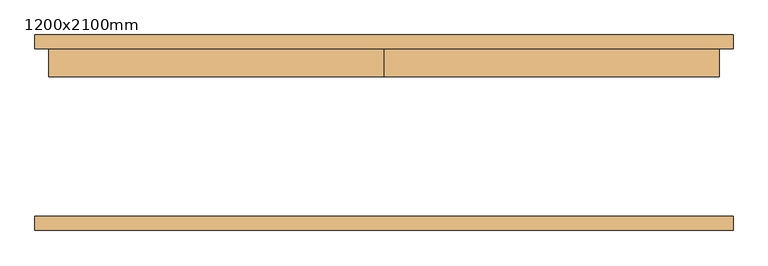
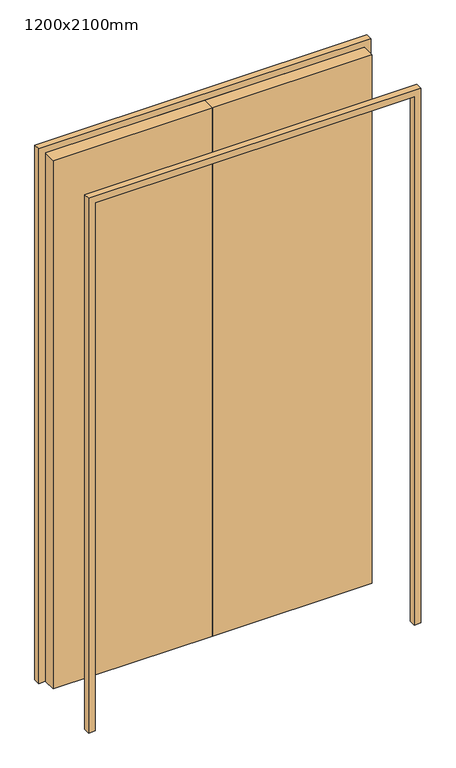
"""IFC4 building model written with IfcOpenShell, lengths in millimetres: door geometry, WWm-DoubleSolid-Flush : 1200x2100mm."""

from ifc_helpers import new_model, si_unit, frame, origin, origin_with_axes, place, context, project, spatial, polyline, outline, extrude, source, transform, mapped, element, save


def door_1200x2100mm_805ceeaa(model_context):
    return source(origin(), model_context, "Body", "SweptSolid", [
        extrude(outline(polyline([(0.0, 150.0), (600.0, 150.0), (600.0, 100.0), (0.0, 100.0), (0.0, 150.0)])), origin_with_axes(), (0.0, 0.0, 1.0), 2100.0),
        extrude(outline(polyline([(-600.0, 150.0), (0.0, 150.0), (0.0, 100.0), (-600.0, 100.0), (-600.0, 150.0)])), origin_with_axes(), (0.0, 0.0, 1.0), 2100.0),
        extrude(outline(polyline([(2100.0, -600.0), (2100.0, 600.0), (0.0, 600.0), (0.0, 625.0), (2125.0, 625.0), (2125.0, -625.0), (0.0, -625.0), (0.0, -600.0), (2100.0, -600.0)])), frame((0.0, -175.0, 0.0), z_axis=(0.0, 1.0, 0.0), x_axis=(0.0, 0.0, 1.0)), (0.0, 0.0, 1.0), 25.0),
        extrude(outline(polyline([(2100.0, -600.0), (2100.0, 600.0), (0.0, 600.0), (0.0, 625.0), (2125.0, 625.0), (2125.0, -625.0), (0.0, -625.0), (0.0, -600.0), (2100.0, -600.0)])), frame((0.0, 150.0, 0.0), z_axis=(0.0, 1.0, 0.0), x_axis=(0.0, 0.0, 1.0)), (0.0, 0.0, 1.0), 25.0),
    ])


if __name__ == "__main__":
    model = new_model("IFC4")
    model_context = context("Model", 3, world=origin())
    ifc_project = project(units=[si_unit("LENGTHUNIT", "METRE", prefix="MILLI")], contexts=[model_context])
    site = spatial("IfcSite", under=ifc_project)
    building = spatial("IfcBuilding", under=site)
    placement = place(None, origin())
    door_1200x2100mm_shape = door_1200x2100mm_805ceeaa(model_context)
    element("IfcDoor", 1, ObjectType="WWm-DoubleSolid-Flush : 1200x2100mm", at=placement, inside=building, context=model_context, shape_type="MappedRepresentation", body=[
        mapped(door_1200x2100mm_shape, transform((0.0, 0.0, 0.0), x_axis=(1.0, 0.0, 0.0), y_axis=(0.0, 1.0, 0.0), z_axis=(0.0, 0.0, 1.0))),
    ])
    save(model, "model.ifc")

# Revit data of these elements
# Type "WWm-DoubleSolid-Flush : 1200x2100mm"
#   Type Mark = "EX1-41"
#   Construction Type Id = "MDOOR"
#   Assembly Code = "C1020"
#   Analytic Construction = "Metal"
#   Thickness = 50 mm
#   Thermal Resistance (R) = 0.270117 (m²·K)/W
#   Heat Transfer Coefficient (U) = 3.7021 W/(m²·K)
#   Height = 2100 mm
#   Trim Projection Ext = 25 mm
#   Trim Projection Int = 25 mm
#   Trim Width = 25 mm
#   Width = 1200 mm
#   Not 90 Degree [instance default] = no
#   90 Degree [instance default] = yes
#   Door Material = WW-EC-RGB-White
#   Frame Material = WW-EC-RGB-White
#   Visual Light Transmittance = 0
#   Solar Heat Gain Coefficient = 0
#   Function = (empty or 0)
#   Wall Closure = (empty or 0)
# Element 1 (IfcDoor, "WWm-DoubleSolid-Flush : 1200x2100mm")
#   Materials on its faces: "WW-EC-RGB-White"
# Materials
#   "WW-EC-RGB-White": class "Generic", colour RGB 255 255 255, transparency 0, Comments = "If region requests off-white, swith asset color to RGB 231-228-220", Description = "Generic Color", Cost = 0
